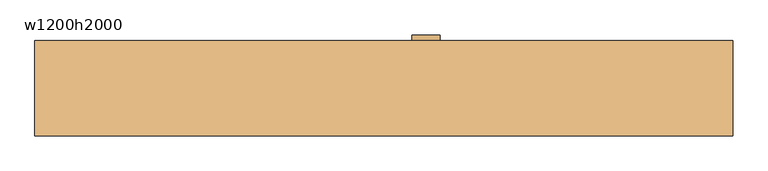
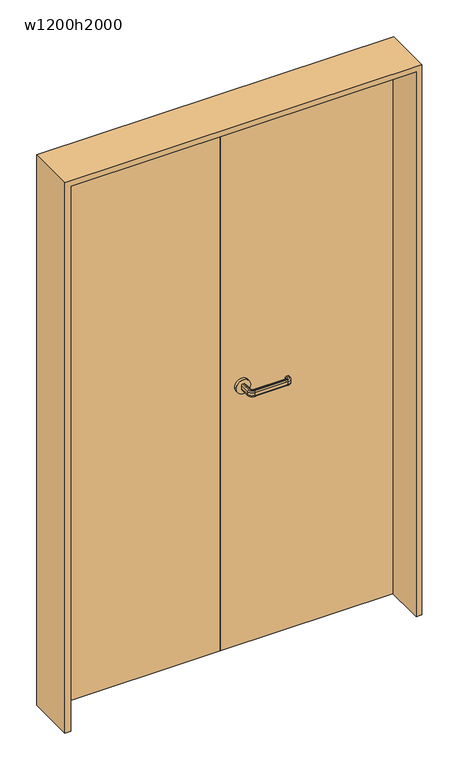
"""IFC4 building model written with IfcOpenShell, lengths in millimetres: door geometry, 二重 : w1200h2000."""

from ifc_helpers import new_model, si_unit, point, frame, frame_2d, origin, origin_with_axes, place, context, project, spatial, polyline, circle_curve, ellipse_curve, trimmed, segment, composite_curve, outline, extrude, source, transform, mapped, element, save
from ifc_brep_helpers import plane_surface, cylinder_surface, revolved_surface, advanced_brep


def w1200h2000_188c20af(model_context):
    return source(origin(), model_context, "Body", "SolidModel", [
        advanced_brep(
        [(77.0, 45.0, 940.0), (73.0, 45.0, 940.0), (68.0, 45.0, 945.0), (68.0, 45.0, 955.0), (73.0, 45.0, 960.0), (77.0, 45.0, 960.0), (82.0, 45.0, 955.0), (82.0, 45.0, 945.0), (77.0, 10.0, 940.0), (85.0, 2.0, 940.0), (200.0, 2.0, 940.0), (208.0, 10.0, 940.0), (208.0, 15.0, 940.0), (212.0, 15.0, 940.0), (212.0, 10.0, 940.0), (200.0, -2.0, 940.0), (85.0, -2.0, 940.0), (73.0, 10.0, 940.0), (68.0, 10.0, 945.0), (68.0, 10.0, 955.0), (73.0, 10.0, 960.0), (85.0, -2.0, 960.0), (200.0, -2.0, 960.0), (212.0, 10.0, 960.0), (212.0, 15.0, 960.0), (208.0, 15.0, 960.0), (208.0, 10.0, 960.0), (200.0, 2.0, 960.0), (85.0, 2.0, 960.0), (77.0, 10.0, 960.0), (82.0, 10.0, 955.0), (82.0, 10.0, 945.0), (85.0, -7.0, 945.0), (85.0, -7.0, 955.0), (85.0, 7.0, 955.0), (85.0, 7.0, 945.0), (200.0, -7.0, 945.0), (200.0, -7.0, 955.0), (200.0, 7.0, 955.0), (200.0, 7.0, 945.0), (217.0, 10.0, 945.0), (217.0, 10.0, 955.0), (203.0, 10.0, 955.0), (203.0, 10.0, 945.0), (203.0, 15.0, 945.0), (203.0, 15.0, 955.0), (217.0, 15.0, 955.0), (217.0, 15.0, 945.0)],
        [
            (0, 1),
            (1, 2, circle_curve(frame((73.0, 45.0, 945.0), z_axis=(0.0, 1.0, 0.0), x_axis=(1.0, 0.0, 0.0)), 5.0)),
            (2, 3),
            (3, 4, circle_curve(frame((73.0, 45.0, 955.0), z_axis=(0.0, 1.0, 0.0), x_axis=(1.0, 0.0, 0.0)), 5.0)),
            (4, 5),
            (5, 6, circle_curve(frame((77.0, 45.0, 955.0), z_axis=(0.0, 1.0, 0.0), x_axis=(1.0, 0.0, 0.0)), 5.0)),
            (6, 7),
            (7, 0, circle_curve(frame((77.0, 45.0, 945.0), z_axis=(0.0, 1.0, 0.0), x_axis=(1.0, 0.0, 0.0)), 5.0)),
            (0, 8),
            (8, 9, circle_curve(frame((85.0, 10.0, 940.0), z_axis=(0.0, 0.0, 1.0), x_axis=(-1.0, 0.0, 0.0)), 8.0)),
            (9, 10),
            (10, 11, circle_curve(frame((200.0, 10.0, 940.0), z_axis=(0.0, 0.0, 1.0), x_axis=(0.0, -1.0, 0.0)), 8.0)),
            (11, 12),
            (12, 13),
            (13, 14),
            (14, 15, circle_curve(frame((200.0, 10.0, 940.0), z_axis=(0.0, 0.0, -1.0), x_axis=(0.0, -1.0, 0.0)), 12.0)),
            (15, 16),
            (16, 17, circle_curve(frame((85.0, 10.0, 940.0), z_axis=(0.0, 0.0, -1.0), x_axis=(-1.0, 0.0, 0.0)), 12.0)),
            (17, 1),
            (17, 18, circle_curve(frame((73.0, 10.0, 945.0), z_axis=(0.0, 1.0, 0.0), x_axis=(1.0, 0.0, 0.0)), 5.0)),
            (18, 2),
            (18, 19),
            (19, 3),
            (19, 20, circle_curve(frame((73.0, 10.0, 955.0), z_axis=(0.0, 1.0, 0.0), x_axis=(1.0, 0.0, 0.0)), 5.0)),
            (20, 4),
            (20, 21, circle_curve(frame((85.0, 10.0, 960.0), z_axis=(0.0, 0.0, 1.0), x_axis=(-1.0, 0.0, 0.0)), 12.0)),
            (21, 22),
            (22, 23, circle_curve(frame((200.0, 10.0, 960.0), z_axis=(0.0, 0.0, 1.0), x_axis=(0.0, -1.0, 0.0)), 12.0)),
            (23, 24),
            (24, 25),
            (25, 26),
            (26, 27, circle_curve(frame((200.0, 10.0, 960.0), z_axis=(0.0, 0.0, -1.0), x_axis=(0.0, -1.0, 0.0)), 8.0)),
            (27, 28),
            (28, 29, circle_curve(frame((85.0, 10.0, 960.0), z_axis=(0.0, 0.0, -1.0), x_axis=(-1.0, 0.0, 0.0)), 8.0)),
            (29, 5),
            (29, 30, circle_curve(frame((77.0, 10.0, 955.0), z_axis=(0.0, 1.0, 0.0), x_axis=(1.0, 0.0, 0.0)), 5.0)),
            (30, 6),
            (30, 31),
            (31, 7),
            (31, 8, circle_curve(frame((77.0, 10.0, 945.0), z_axis=(0.0, 1.0, 0.0), x_axis=(1.0, 0.0, 0.0)), 5.0)),
            (32, 18, circle_curve(frame((85.0, 10.0, 945.0), z_axis=(0.0, 0.0, -1.0), x_axis=(-1.0, 0.0, 0.0)), 17.0)),
            (16, 32, circle_curve(frame((85.0, -2.0, 945.0), z_axis=(-1.0, 0.0, 0.0), x_axis=(0.0, 1.0, 0.0)), 5.0)),
            (33, 19, circle_curve(frame((85.0, 10.0, 955.0), z_axis=(0.0, 0.0, -1.0), x_axis=(-1.0, 0.0, 0.0)), 17.0)),
            (32, 33),
            (33, 21, circle_curve(frame((85.0, -2.0, 955.0), z_axis=(-1.0, 0.0, 0.0), x_axis=(0.0, 1.0, 0.0)), 5.0)),
            (34, 30, circle_curve(frame((85.0, 10.0, 955.0), z_axis=(0.0, 0.0, -1.0), x_axis=(-1.0, 0.0, 0.0)), 3.0)),
            (28, 34, circle_curve(frame((85.0, 2.0, 955.0), z_axis=(-1.0, 0.0, 0.0), x_axis=(0.0, 1.0, 0.0)), 5.0)),
            (35, 31, circle_curve(frame((85.0, 10.0, 945.0), z_axis=(0.0, 0.0, -1.0), x_axis=(-1.0, 0.0, 0.0)), 3.0)),
            (34, 35),
            (35, 9, circle_curve(frame((85.0, 2.0, 945.0), z_axis=(-1.0, 0.0, 0.0), x_axis=(0.0, 1.0, 0.0)), 5.0)),
            (15, 36, circle_curve(frame((200.0, -2.0, 945.0), z_axis=(-1.0, 0.0, 0.0), x_axis=(0.0, 1.0, 0.0)), 5.0)),
            (36, 32),
            (36, 37),
            (37, 33),
            (37, 22, circle_curve(frame((200.0, -2.0, 955.0), z_axis=(-1.0, 0.0, 0.0), x_axis=(0.0, 1.0, 0.0)), 5.0)),
            (27, 38, circle_curve(frame((200.0, 2.0, 955.0), z_axis=(-1.0, 0.0, 0.0), x_axis=(0.0, 1.0, 0.0)), 5.0)),
            (38, 34),
            (38, 39),
            (39, 35),
            (39, 10, circle_curve(frame((200.0, 2.0, 945.0), z_axis=(-1.0, 0.0, 0.0), x_axis=(0.0, 1.0, 0.0)), 5.0)),
            (40, 36, circle_curve(frame((200.0, 10.0, 945.0), z_axis=(0.0, 0.0, -1.0), x_axis=(0.0, -1.0, 0.0)), 17.0)),
            (14, 40, circle_curve(frame((212.0, 10.0, 945.0), z_axis=(0.0, -1.0, 0.0), x_axis=(-1.0, 0.0, 0.0)), 5.0)),
            (41, 37, circle_curve(frame((200.0, 10.0, 955.0), z_axis=(0.0, 0.0, -1.0), x_axis=(0.0, -1.0, 0.0)), 17.0)),
            (40, 41),
            (41, 23, circle_curve(frame((212.0, 10.0, 955.0), z_axis=(0.0, -1.0, 0.0), x_axis=(-1.0, 0.0, 0.0)), 5.0)),
            (42, 38, circle_curve(frame((200.0, 10.0, 955.0), z_axis=(0.0, 0.0, -1.0), x_axis=(0.0, -1.0, 0.0)), 3.0)),
            (26, 42, circle_curve(frame((208.0, 10.0, 955.0), z_axis=(0.0, -1.0, 0.0), x_axis=(-1.0, 0.0, 0.0)), 5.0)),
            (43, 39, circle_curve(frame((200.0, 10.0, 945.0), z_axis=(0.0, 0.0, -1.0), x_axis=(0.0, -1.0, 0.0)), 3.0)),
            (42, 43),
            (43, 11, circle_curve(frame((208.0, 10.0, 945.0), z_axis=(0.0, -1.0, 0.0), x_axis=(-1.0, 0.0, 0.0)), 5.0)),
            (12, 44, circle_curve(frame((208.0, 15.0, 945.0), z_axis=(0.0, 1.0, 0.0), x_axis=(-1.0, 0.0, 0.0)), 5.0)),
            (44, 45),
            (45, 25, circle_curve(frame((208.0, 15.0, 955.0), z_axis=(0.0, 1.0, 0.0), x_axis=(-1.0, 0.0, 0.0)), 5.0)),
            (24, 46, circle_curve(frame((212.0, 15.0, 955.0), z_axis=(0.0, 1.0, 0.0), x_axis=(-1.0, 0.0, 0.0)), 5.0)),
            (46, 47),
            (47, 13, circle_curve(frame((212.0, 15.0, 945.0), z_axis=(0.0, 1.0, 0.0), x_axis=(-1.0, 0.0, 0.0)), 5.0)),
            (47, 40),
            (46, 41),
            (45, 42),
            (44, 43),
        ],
        [
            plane_surface(frame((64.801961, 45.0, 950.0), z_axis=(0.0, 1.0, 0.0), x_axis=(0.0, 0.0, -1.0))),
            plane_surface(frame((77.0, 45.0, 940.0), z_axis=(0.0, 0.0, -1.0), x_axis=(0.0, -1.0, 0.0))),
            cylinder_surface(frame((73.0, 45.0, 945.0), z_axis=(0.0, 1.0, 0.0), x_axis=(1.0, 0.0, 0.0)), 5.0),
            plane_surface(frame((68.0, 45.0, 945.0), z_axis=(-1.0, 0.0, 0.0), x_axis=(0.0, -1.0, 0.0))),
            cylinder_surface(frame((73.0, 45.0, 955.0), z_axis=(0.0, 1.0, 0.0), x_axis=(1.0, 0.0, 0.0)), 5.0),
            plane_surface(frame((73.0, 45.0, 960.0), z_axis=(0.0, 0.0, 1.0), x_axis=(0.0, -1.0, 0.0))),
            cylinder_surface(frame((77.0, 45.0, 955.0), z_axis=(0.0, 1.0, 0.0), x_axis=(1.0, 0.0, 0.0)), 5.0),
            plane_surface(frame((82.0, 45.0, 955.0), z_axis=(1.0, 0.0, 0.0), x_axis=(0.0, -1.0, 0.0))),
            cylinder_surface(frame((77.0, 45.0, 945.0), z_axis=(0.0, 1.0, 0.0), x_axis=(1.0, 0.0, 0.0)), 5.0),
            revolved_surface(trimmed(ellipse_curve(frame((73.0, 10.0, 945.0), z_axis=(0.0, 1.0, 0.0), x_axis=(1.0, 0.0, 0.0)), 5.0, 5.0), [point((73.0, 10.0, 940.0))], [point((68.0, 10.0, 945.0))], True, "CARTESIAN"), (85.0, 10.0, 950.0), (0.0, 0.0, 1.0)),
            cylinder_surface(frame((85.0, 10.0, 950.0), z_axis=(0.0, 0.0, 1.0), x_axis=(-1.0, 0.0, 0.0)), 17.0),
            revolved_surface(trimmed(ellipse_curve(frame((73.0, 10.0, 955.0), z_axis=(0.0, 1.0, 0.0), x_axis=(1.0, 0.0, 0.0)), 5.0, 5.0), [point((68.0, 10.0, 955.0))], [point((73.0, 10.0, 960.0))], True, "CARTESIAN"), (85.0, 10.0, 950.0), (0.0, 0.0, 1.0)),
            revolved_surface(trimmed(ellipse_curve(frame((77.0, 10.0, 955.0), z_axis=(0.0, 1.0, 0.0), x_axis=(1.0, 0.0, 0.0)), 5.0, 5.0), [point((77.0, 10.0, 960.0))], [point((82.0, 10.0, 955.0))], True, "CARTESIAN"), (85.0, 10.0, 950.0), (0.0, 0.0, 1.0)),
            revolved_surface(polyline([(82.0, 10.0, 955.0), (82.0, 10.0, 945.0)]), (85.0, 10.0, 950.0), (0.0, 0.0, 1.0)),
            revolved_surface(trimmed(ellipse_curve(frame((77.0, 10.0, 945.0), z_axis=(0.0, 1.0, 0.0), x_axis=(1.0, 0.0, 0.0)), 5.0, 5.0), [point((82.0, 10.0, 945.0))], [point((77.0, 10.0, 940.0))], True, "CARTESIAN"), (85.0, 10.0, 950.0), (0.0, 0.0, 1.0)),
            cylinder_surface(frame((85.0, -2.0, 945.0), z_axis=(-1.0, 0.0, 0.0), x_axis=(0.0, 1.0, 0.0)), 5.0),
            plane_surface(frame((85.0, -7.0, 945.0), z_axis=(0.0, -1.0, 0.0), x_axis=(1.0, 0.0, 0.0))),
            cylinder_surface(frame((85.0, -2.0, 955.0), z_axis=(-1.0, 0.0, 0.0), x_axis=(0.0, 1.0, 0.0)), 5.0),
            cylinder_surface(frame((85.0, 2.0, 955.0), z_axis=(-1.0, 0.0, 0.0), x_axis=(0.0, 1.0, 0.0)), 5.0),
            plane_surface(frame((85.0, 7.0, 955.0), z_axis=(0.0, 1.0, 0.0), x_axis=(1.0, 0.0, 0.0))),
            cylinder_surface(frame((85.0, 2.0, 945.0), z_axis=(-1.0, 0.0, 0.0), x_axis=(0.0, 1.0, 0.0)), 5.0),
            revolved_surface(trimmed(ellipse_curve(frame((200.0, -2.0, 945.0), z_axis=(-1.0, 0.0, 0.0), x_axis=(0.0, 1.0, 0.0)), 5.0, 5.0), [point((200.0, -2.0, 940.0))], [point((200.0, -7.0, 945.0))], True, "CARTESIAN"), (200.0, 10.0, 950.0), (0.0, 0.0, 1.0)),
            cylinder_surface(frame((200.0, 10.0, 950.0), z_axis=(0.0, 0.0, 1.0), x_axis=(0.0, -1.0, 0.0)), 17.0),
            revolved_surface(trimmed(ellipse_curve(frame((200.0, -2.0, 955.0), z_axis=(-1.0, 0.0, 0.0), x_axis=(0.0, 1.0, 0.0)), 5.0, 5.0), [point((200.0, -7.0, 955.0))], [point((200.0, -2.0, 960.0))], True, "CARTESIAN"), (200.0, 10.0, 950.0), (0.0, 0.0, 1.0)),
            revolved_surface(trimmed(ellipse_curve(frame((200.0, 2.0, 955.0), z_axis=(-1.0, 0.0, 0.0), x_axis=(0.0, 1.0, 0.0)), 5.0, 5.0), [point((200.0, 2.0, 960.0))], [point((200.0, 7.0, 955.0))], True, "CARTESIAN"), (200.0, 10.0, 950.0), (0.0, 0.0, 1.0)),
            revolved_surface(polyline([(200.0, 7.0, 955.0), (200.0, 7.0, 945.0)]), (200.0, 10.0, 950.0), (0.0, 0.0, 1.0)),
            revolved_surface(trimmed(ellipse_curve(frame((200.0, 2.0, 945.0), z_axis=(-1.0, 0.0, 0.0), x_axis=(0.0, 1.0, 0.0)), 5.0, 5.0), [point((200.0, 7.0, 945.0))], [point((200.0, 2.0, 940.0))], True, "CARTESIAN"), (200.0, 10.0, 950.0), (0.0, 0.0, 1.0)),
            plane_surface(frame((199.801961, 15.0, 950.0), z_axis=(0.0, 1.0, 0.0), x_axis=(0.0, 0.0, 1.0))),
            cylinder_surface(frame((212.0, 10.0, 945.0), z_axis=(0.0, -1.0, 0.0), x_axis=(-1.0, 0.0, 0.0)), 5.0),
            plane_surface(frame((217.0, 10.0, 945.0), z_axis=(1.0, 0.0, 0.0), x_axis=(0.0, 1.0, 0.0))),
            cylinder_surface(frame((212.0, 10.0, 955.0), z_axis=(0.0, -1.0, 0.0), x_axis=(-1.0, 0.0, 0.0)), 5.0),
            cylinder_surface(frame((208.0, 10.0, 955.0), z_axis=(0.0, -1.0, 0.0), x_axis=(-1.0, 0.0, 0.0)), 5.0),
            plane_surface(frame((203.0, 10.0, 955.0), z_axis=(-1.0, 0.0, 0.0), x_axis=(0.0, 1.0, 0.0))),
            cylinder_surface(frame((208.0, 10.0, 945.0), z_axis=(0.0, -1.0, 0.0), x_axis=(-1.0, 0.0, 0.0)), 5.0),
        ],
        [
            (0, [[1, 2, 3, 4, 5, 6, 7, 8]]),
            (1, [[-1, 9, 10, 11, 12, 13, 14, 15, 16, 17, 18, 19]]),
            (2, [[-2, -19, 20, 21]]),
            (3, [[-3, -21, 22, 23]]),
            (4, [[-4, -23, 24, 25]]),
            (5, [[-5, -25, 26, 27, 28, 29, 30, 31, 32, 33, 34, 35]]),
            (6, [[-6, -35, 36, 37]]),
            (7, [[-7, -37, 38, 39]]),
            (8, [[-8, -39, 40, -9]]),
            (9, [[41, -20, -18, 42]]),
            (10, [[43, -22, -41, 44]]),
            (11, [[-26, -24, -43, 45]]),
            (12, [[46, -36, -34, 47]]),
            (13, [[48, -38, -46, 49]]),
            (14, [[-10, -40, -48, 50]]),
            (15, [[-42, -17, 51, 52]]),
            (16, [[-44, -52, 53, 54]]),
            (17, [[-45, -54, 55, -27]]),
            (18, [[-47, -33, 56, 57]]),
            (19, [[-49, -57, 58, 59]]),
            (20, [[-50, -59, 60, -11]]),
            (21, [[61, -51, -16, 62]]),
            (22, [[63, -53, -61, 64]]),
            (23, [[-28, -55, -63, 65]]),
            (24, [[66, -56, -32, 67]]),
            (25, [[68, -58, -66, 69]]),
            (26, [[-12, -60, -68, 70]]),
            (27, [[71, 72, 73, -30, 74, 75, 76, -14]]),
            (28, [[-62, -15, -76, 77]]),
            (29, [[-64, -77, -75, 78]]),
            (30, [[-65, -78, -74, -29]]),
            (31, [[-67, -31, -73, 79]]),
            (32, [[-69, -79, -72, 80]]),
            (33, [[-70, -80, -71, -13]]),
        ],
    ),
        extrude(outline(composite_curve([segment(trimmed(circle_curve(frame_2d((950.0, 75.0)), 25.0), [point((950.0, 50.0))], [point((950.0, 100.0))], False, "CARTESIAN"), True, "CONTINUOUS"), segment(trimmed(circle_curve(frame_2d((950.0, 75.0)), 25.0), [point((950.0, 100.0))], [point((950.0, 50.0))], False, "CARTESIAN"), True, "CONTINUOUS")], self_intersect=False)), frame((0.0, 85.0, 0.0), z_axis=(0.0, 1.0, 0.0), x_axis=(0.0, 0.0, 1.0)), (0.0, 0.0, 1.0), 10.0),
        extrude(outline(composite_curve([segment(trimmed(circle_curve(frame_2d((950.0, 75.0)), 25.0), [point((950.0, 50.0))], [point((950.0, 100.0))], False, "CARTESIAN"), True, "CONTINUOUS"), segment(trimmed(circle_curve(frame_2d((950.0, 75.0)), 25.0), [point((950.0, 100.0))], [point((950.0, 50.0))], False, "CARTESIAN"), True, "CONTINUOUS")], self_intersect=False)), frame((0.0, 45.0, 0.0), z_axis=(0.0, 1.0, 0.0), x_axis=(0.0, 0.0, 1.0)), (0.0, 0.0, 1.0), 10.0),
        extrude(outline(polyline([(0.0, 55.0), (-600.0, 55.0), (-600.0, 85.0), (0.0, 85.0), (0.0, 55.0)])), origin_with_axes(), (0.0, 0.0, 1.0), 2000.0),
        extrude(outline(polyline([(2020.0, -620.0), (0.0, -620.0), (0.0, -600.0), (2000.0, -600.0), (2000.0, 600.0), (0.0, 600.0), (0.0, 620.0), (2020.0, 620.0), (2020.0, -620.0)])), frame((0.0, -85.0, 0.0), z_axis=(0.0, 1.0, 0.0), x_axis=(0.0, 0.0, 1.0)), (0.0, 0.0, 1.0), 170.0),
        extrude(outline(polyline([(600.0, 55.0), (0.0, 55.0), (0.0, 85.0), (600.0, 85.0), (600.0, 55.0)])), origin_with_axes(), (0.0, 0.0, 1.0), 2000.0),
    ])


if __name__ == "__main__":
    model = new_model("IFC4")
    model_context = context("Model", 3, world=origin())
    ifc_project = project(units=[si_unit("LENGTHUNIT", "METRE", prefix="MILLI")], contexts=[model_context])
    site = spatial("IfcSite", under=ifc_project)
    building = spatial("IfcBuilding", under=site)
    placement = place(None, origin())
    w1200h2000_shape = w1200h2000_188c20af(model_context)
    element("IfcDoor", 1, ObjectType="二重 : w1200h2000", at=placement, inside=building, context=model_context, shape_type="MappedRepresentation", body=[
        mapped(w1200h2000_shape, transform((0.0, 0.0, 0.0), x_axis=(1.0, 0.0, 0.0), y_axis=(0.0, 1.0, 0.0), z_axis=(0.0, 0.0, 1.0))),
    ])
    save(model, "model.ifc")

# Revit data of these elements
# Type "二重 : w1200h2000"
#   Construction Type Id = "MDOOR"
#   Analytic Construction = "メタル"
#   Type Mark = "47"
#   Operation = "両開きドア単一スイング"
#   Keynote = "08110.R1"
#   Visual Light Transmittance = 0
#   Solar Heat Gain Coefficient = 0
#   Heat Transfer Coefficient (U) = 3.7021 W/(m²·K)
#   高さ(中心) = 1000 mm
#   Height = 2000 mm
#   Thickness = 30 mm
#   ドア枠見附 = 20 mm
#   Width = 1200 mm
#   取手取付け高さ = 950 mm
#   ドア枠ちり = 10 mm
#   Function = 0
#   ドア枠 [instance default] = none
#   ドア把手 [instance default] = メタル-ステンレス
#   ドア [instance default] = none
#   Wall Closure = (empty or 0)
# Element 1 (IfcDoor, "二重 : w1200h2000")
#   Materials on its faces: "メタル-ステンレス"
# Materials
#   "メタル-ステンレス": class "メタル", colour RGB 247 247 247, transparency 0, Cost = 0
